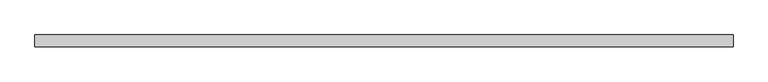
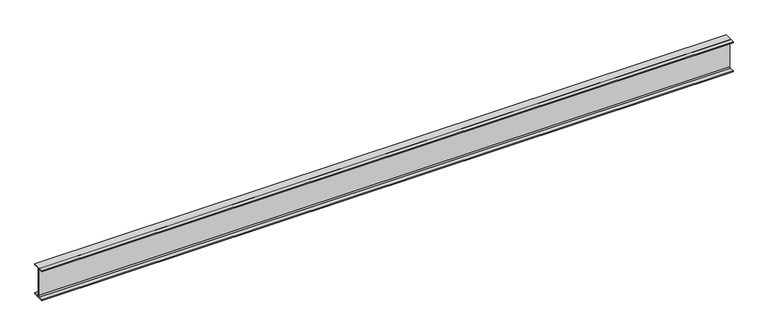
"""IFC4 building model written with IfcOpenShell, lengths in millimetres: beam geometry, Steel Framing_H_KS : H_SB_AR_S02_H-800x300x14x26_SRG1."""

from ifc_helpers import new_model, si_unit, point, frame, frame_2d, origin, place, context, project, spatial, polyline, circle_curve, trimmed, segment, composite_curve, outline, extrude, source, transform, mapped, element, save


def beam_a13b9fc3(model_context):
    return source(origin(), model_context, "Body", "SweptSolid", [
        extrude(outline(composite_curve([segment(polyline([(150.0, -374.0), (150.0, -400.0), (-150.0, -400.0), (-150.0, -374.0), (-35.0, -374.0)]), True, "CONTINUOUS"), segment(trimmed(circle_curve(frame_2d((-35.0, -346.0)), 28.0), [point((-35.0, -374.0))], [point((-7.0, -346.0))], True, "CARTESIAN"), True, "CONTINUOUS"), segment(polyline([(-7.0, -346.0), (-7.0, 346.0)]), True, "CONTINUOUS"), segment(trimmed(circle_curve(frame_2d((-35.0, 346.0)), 28.0), [point((-7.0, 346.0))], [point((-35.0, 374.0))], True, "CARTESIAN"), True, "CONTINUOUS"), segment(polyline([(-35.0, 374.0), (-150.0, 374.0), (-150.0, 400.0), (150.0, 400.0), (150.0, 374.0), (35.0, 374.0)]), True, "CONTINUOUS"), segment(trimmed(circle_curve(frame_2d((35.0, 346.0)), 28.0), [point((35.0, 374.0))], [point((7.0, 346.0))], True, "CARTESIAN"), True, "CONTINUOUS"), segment(polyline([(7.0, 346.0), (7.0, -346.0)]), True, "CONTINUOUS"), segment(trimmed(circle_curve(frame_2d((35.0, -346.0)), 28.0), [point((7.0, -346.0))], [point((35.0, -374.0))], True, "CARTESIAN"), True, "CONTINUOUS"), segment(polyline([(35.0, -374.0), (150.0, -374.0)]), True, "CONTINUOUS")], self_intersect=False)), frame((-8693.3, 0.0, 0.0), z_axis=(1.0, 0.0, 0.0), x_axis=(0.0, 1.0, 0.0)), (0.0, 0.0, 1.0), 17386.6),
    ])


if __name__ == "__main__":
    model = new_model("IFC4")
    model_context = context("Model", 3, world=origin())
    ifc_project = project(units=[si_unit("LENGTHUNIT", "METRE", prefix="MILLI")], contexts=[model_context])
    site = spatial("IfcSite", under=ifc_project)
    building = spatial("IfcBuilding", under=site)
    placement = place(None, origin())
    beam_shape = beam_a13b9fc3(model_context)
    element("IfcBeam", 1, ObjectType="Steel Framing_H_KS : H_SB_AR_S02_H-800x300x14x26_SRG1", at=placement, inside=building, context=model_context, shape_type="MappedRepresentation", body=[
        mapped(beam_shape, transform((0.0, 0.0, 0.0), x_axis=(1.0, 0.0, 0.0), y_axis=(0.0, 1.0, 0.0), z_axis=(0.0, 0.0, 1.0))),
    ])
    save(model, "model.ifc")

# Revit data of these elements
# Type "Steel Framing_H_KS : H_SB_AR_S02_H-800x300x14x26_SRG1"
#   Type Comments = "MAIN"
#   Type Mark = "SRG1"
#   H_SectionID = "H-800x300x14x26"
#   H_Ratio for Additional Steel Plate = 0.2
#   Width = 30.0 cm
#   Web Thickness = 1.4 cm
#   Web Fillet = 2.8 cm
#   Warping Constant = 17500000.0 cm⁶
#   Torsional Moment of Inertia = 422.315 cm⁴
#   Section Area = 267.4 cm²
#   Plastic Modulus weak axis = 1220.0 cm³
#   Plastic Modulus strong axis = 8240.0 cm³
#   Perimeter = 2.72 m²/m
#   Nominal Weight = 210.00 kgf/m
#   Moment of Inertia weak axis = 11700.00 cm⁴
#   Moment of Inertia strong axis = 292000.00 cm⁴
#   Height = 80.0 cm
#   Flange Thickness = 2.6 cm
#   Elastic Modulus weak axis = 782.0 cm³
#   Elastic Modulus strong axis = 7290.0 cm³
#   Centroid Vertical = 40.0 cm
#   Centroid Horizontal = 15.0 cm
#   Bolt Spacing = 8.89 cm
#   Length [instance default] = 1500 mm
#   Structural Material [instance default] = Steel, 45-345
#   Section Name Key = ""
#   Assembly Code = ""
# Element 1 (IfcBeam, "Steel Framing_H_KS : H_SB_AR_S02_H-800x300x14x26_SRG1")
#   Materials on its faces: "Steel, 45-345"
# Materials
#   "Steel, 45-345": class "Metal", colour RGB 189 187 185, transparency 0, Description = "Steel 345 MPa", Cost = 0
